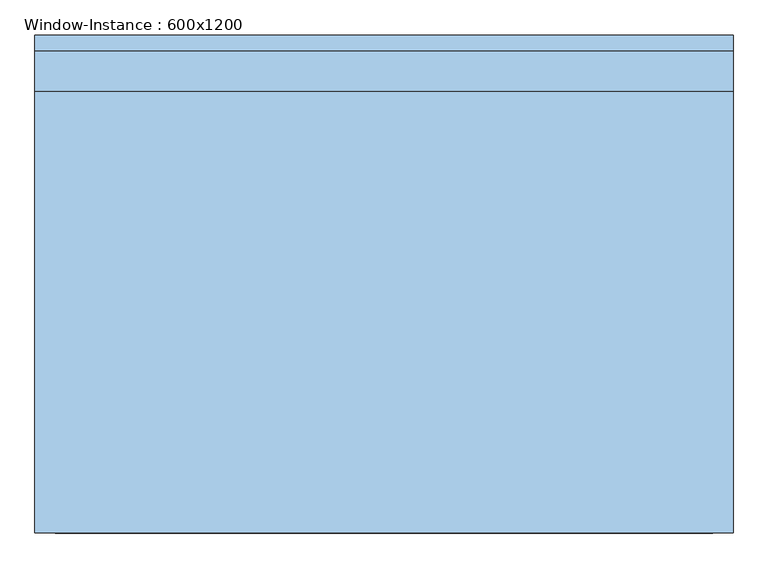
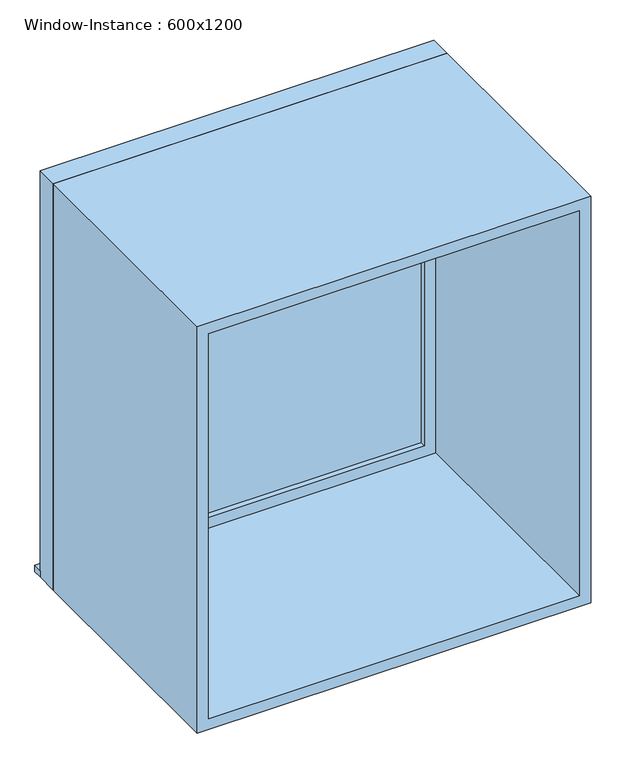
"""IFC4 building model written with IfcOpenShell, lengths in millimetres: window geometry, Window-Instance : 600x1200."""

from ifc_helpers import new_model, si_unit, frame, origin, place, context, project, spatial, polyline, outline, extrude, source, transform, mapped, element, save


def window_instance_600x1200_862d08fa(model_context):
    return source(origin(), model_context, "Body", "SweptSolid", [
        extrude(outline(polyline([(-588.1, 405.4), (511.9, 405.4), (511.9, 380.0), (-588.1, 380.0), (-588.1, 405.4)])), frame((0.0, 0.0, 900.0), z_axis=(0.0, 0.0, 1.0), x_axis=(1.0, 0.0, 0.0)), (0.0, 0.0, 1.0), 19.05),
        extrude(outline(polyline([(448.4, 331.425), (-524.6, 331.425), (-524.6, 344.125), (448.4, 344.125), (448.4, 331.425)])), frame((0.0, 0.0, 963.5), z_axis=(0.0, 0.0, 1.0), x_axis=(1.0, 0.0, 0.0)), (0.0, 0.0, 1.0), 1073.0),
        extrude(outline(polyline([(2080.95, -569.05), (919.05, -569.05), (919.05, 492.85), (2080.95, 492.85), (2080.95, -569.05)]), holes=[polyline([(2036.5, -524.6), (2036.5, 448.4), (963.5, 448.4), (963.5, -524.6), (2036.5, -524.6)])]), frame((0.0, 315.55, 0.0), z_axis=(0.0, 1.0, 0.0), x_axis=(0.0, 0.0, 1.0)), (0.0, 0.0, 1.0), 44.45),
        extrude(outline(polyline([(2100.0, -588.1), (900.0, -588.1), (900.0, 511.9), (2100.0, 511.9), (2100.0, -588.1)]), holes=[polyline([(2068.25, -556.35), (2068.25, 480.15), (931.75, 480.15), (931.75, -556.35), (2068.25, -556.35)])]), frame((0.0, -380.0, 0.0), z_axis=(0.0, 1.0, 0.0), x_axis=(0.0, 0.0, 1.0)), (0.0, 0.0, 1.0), 695.55),
        extrude(outline(polyline([(2100.0, 511.9), (2100.0, -588.1), (900.0, -588.1), (900.0, 511.9), (2100.0, 511.9)]), holes=[polyline([(2080.95, 492.85), (919.05, 492.85), (919.05, -569.05), (2080.95, -569.05), (2080.95, 492.85)])]), frame((0.0, 315.55, 0.0), z_axis=(0.0, 1.0, 0.0), x_axis=(0.0, 0.0, 1.0)), (0.0, 0.0, 1.0), 64.45),
    ])


if __name__ == "__main__":
    model = new_model("IFC4")
    model_context = context("Model", 3, world=origin())
    ifc_project = project(units=[si_unit("LENGTHUNIT", "METRE", prefix="MILLI")], contexts=[model_context])
    site = spatial("IfcSite", under=ifc_project)
    building = spatial("IfcBuilding", under=site)
    placement = place(None, origin())
    window_instance_600x1200_shape = window_instance_600x1200_862d08fa(model_context)
    element("IfcWindow", 1, ObjectType="Window-Instance : 600x1200", at=placement, inside=building, context=model_context, shape_type="MappedRepresentation", body=[
        mapped(window_instance_600x1200_shape, transform((0.0, 0.0, 0.0), x_axis=(1.0, 0.0, 0.0), y_axis=(0.0, 1.0, 0.0), z_axis=(0.0, 0.0, 1.0))),
    ])
    save(model, "model.ifc")

# Revit data of these elements
# Type "Window-Instance : 600x1200"
#   Type Mark = "7"
#   Construction Type Id = "GSP4R"
#   Assembly Code = "B2020100"
#   Analytic Construction = "1/8 in Pilkington single glazing"
#   Visual Light Transmittance = 0.9
#   Thermal Resistance (R) = 0.149095 (m²·K)/W
#   Solar Heat Gain Coefficient = 0.86
#   Heat Transfer Coefficient (U) = 6.70716 W/(m²·K)
#   Height [instance default] = 1200 mm
#   Default Sill Height = 900 mm
#   Width [instance default] = 600 mm
#   Window Inset = 20 mm
#   Glass Pane Material = WW-EC-GL-Storefront
#   Sash Material = WW-EC-RGB-White
#   Wall Closure = (empty or 0)
# Element 1 (IfcWindow, "Window-Instance : 600x1200")
#   Width = 1100 mm
#   Materials on its faces: "WW-EC-RGB-White", "WW-EC-GL-Storefront"
# Materials
#   "WW-EC-GL-Storefront": class "Glass", colour RGB 236 240 239, transparency 0.85, Description = "Storefront Glass", Cost = 0
#   "WW-EC-RGB-White": class "Generic", colour RGB 255 255 255, transparency 0, Comments = "If region requests off-white, swith asset color to RGB 231-228-220", Description = "Generic Color", Cost = 0
